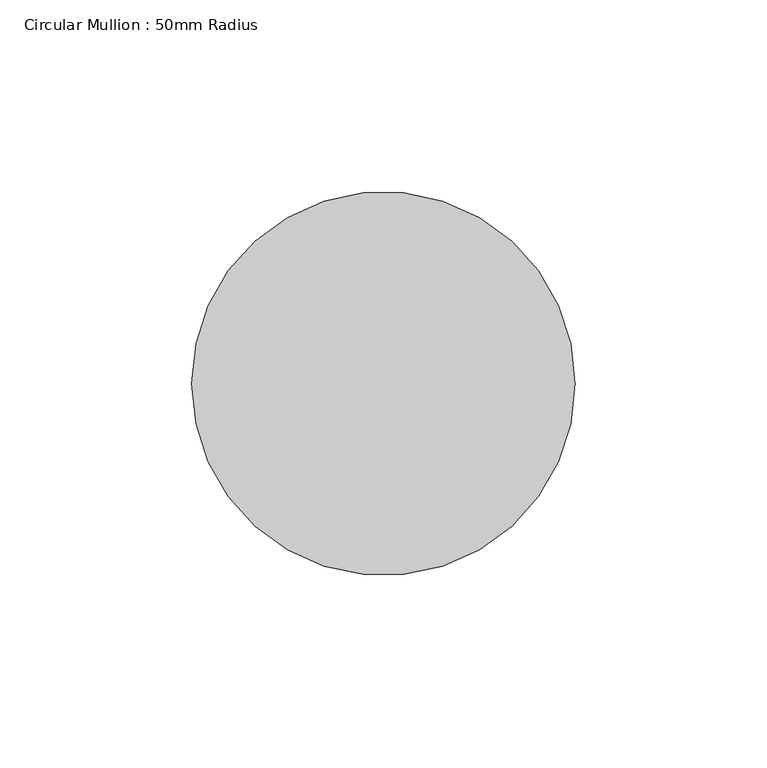
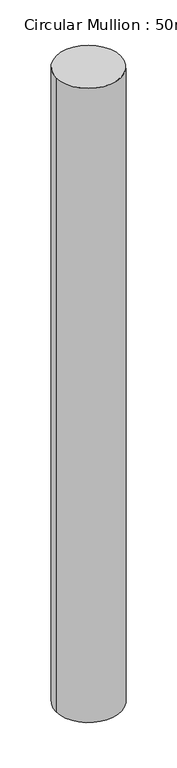
"""IFC4 building model written with IfcOpenShell, lengths in millimetres: member geometry, Circular Mullion : 50mm Radius."""

from ifc_helpers import new_model, si_unit, point, frame, origin, origin_2d, place, context, project, spatial, circle_curve, trimmed, segment, composite_curve, outline, extrude, source, transform, mapped, element, save


def circular_mullion_50mm_radius_4e72ec76(model_context):
    return source(origin(), model_context, "Body", "SweptSolid", [
        extrude(outline(composite_curve([segment(trimmed(circle_curve(origin_2d(), 50.0), [point((50.0, 0.0))], [point((-50.0, 0.0))], False, "CARTESIAN"), True, "CONTINUOUS"), segment(trimmed(circle_curve(origin_2d(), 50.0), [point((-50.0, 0.0))], [point((50.0, 0.0))], False, "CARTESIAN"), True, "CONTINUOUS")], self_intersect=False)), frame((0.0, 0.0, -1032.7186893), z_axis=(0.0, 0.0, 1.0), x_axis=(1.0, 0.0, 0.0)), (0.0, 0.0, 1.0), 1032.7186893),
    ])


if __name__ == "__main__":
    model = new_model("IFC4")
    model_context = context("Model", 3, world=origin())
    ifc_project = project(units=[si_unit("LENGTHUNIT", "METRE", prefix="MILLI")], contexts=[model_context])
    site = spatial("IfcSite", under=ifc_project)
    building = spatial("IfcBuilding", under=site)
    placement = place(None, origin())
    circular_mullion_50mm_radius_shape = circular_mullion_50mm_radius_4e72ec76(model_context)
    element("IfcMember", 1, ObjectType="Circular Mullion : 50mm Radius", at=placement, inside=building, context=model_context, shape_type="MappedRepresentation", body=[
        mapped(circular_mullion_50mm_radius_shape, transform((0.0, 0.0, 0.0), x_axis=(1.0, 0.0, 0.0), y_axis=(0.0, 1.0, 0.0), z_axis=(0.0, 0.0, 1.0))),
    ])
    save(model, "model.ifc")

# Revit data of these elements
# Type "Circular Mullion : 50mm Radius"
#   built-in parameter 1007350 = 0.164042 (stored number, unit not read)
# Element 1 (IfcMember, "Circular Mullion : 50mm Radius")
#   Materials on its faces: "Aluminium"
# Materials
#   "Aluminium": class "Metal", colour RGB 247 247 247, transparency 0, Description = "Aluminium 6061", Cost = 0
